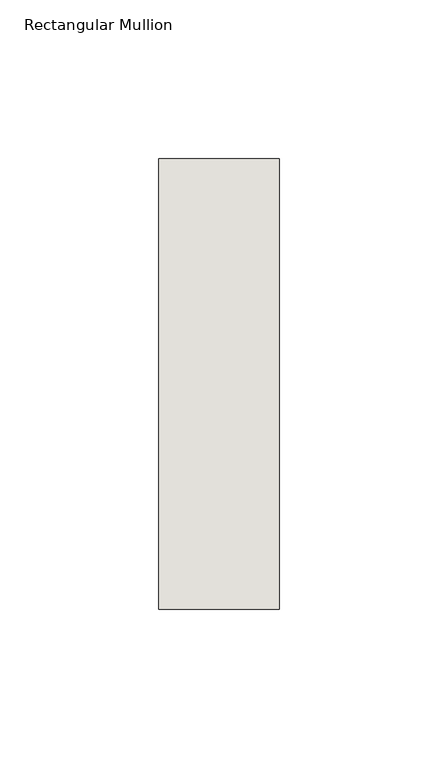
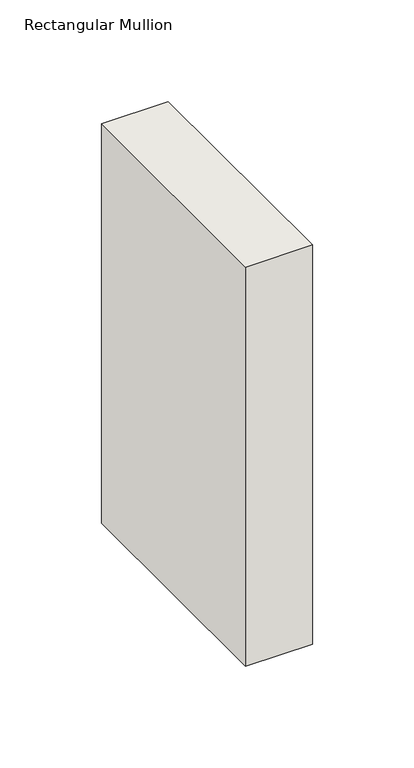
"""IFC4 building model written with IfcOpenShell, lengths in millimetres: wall geometry, Rectangular Mullion : NLRS_21_CWM_hsb-regel 38x142_gen_rsf."""

from ifc_helpers import new_model, si_unit, frame, origin, place, context, project, spatial, polyline, outline, extrude, source, transform, mapped, element, save


def rectangular_mullion_5bdfe98c(model_context):
    return source(origin(), model_context, "Body", "SweptSolid", [
        extrude(outline(polyline([(19.0, -71.0), (-19.0, -71.0), (-19.0, 71.0), (19.0, 71.0), (19.0, -71.0)])), frame((0.0, 0.0, -239.8441061), z_axis=(0.0, 0.0, 1.0), x_axis=(1.0, 0.0, 0.0)), (0.0, 0.0, 1.0), 239.8441061),
    ])


if __name__ == "__main__":
    model = new_model("IFC4")
    model_context = context("Model", 3, world=origin())
    ifc_project = project(units=[si_unit("LENGTHUNIT", "METRE", prefix="MILLI")], contexts=[model_context])
    site = spatial("IfcSite", under=ifc_project)
    building = spatial("IfcBuilding", under=site)
    placement = place(None, origin())
    rectangular_mullion_shape = rectangular_mullion_5bdfe98c(model_context)
    element("IfcWall", 1, ObjectType="Rectangular Mullion : NLRS_21_CWM_hsb-regel 38x142_gen_rsf", at=placement, inside=building, context=model_context, shape_type="MappedRepresentation", body=[
        mapped(rectangular_mullion_shape, transform((0.0, 0.0, 0.0), x_axis=(1.0, 0.0, 0.0), y_axis=(0.0, 1.0, 0.0), z_axis=(0.0, 0.0, 1.0))),
    ])
    save(model, "model.ifc")

# Revit data of these elements
# Type "Rectangular Mullion : NLRS_21_CWM_hsb-regel 38x142_gen_rsf"
#   Type IfcGUID = "07M7mRoiH1CR8m_RSKIwpF"
#   Assembly Code = "21.10"
#   IfcExportAs = "IfcWall"
#   built-in parameter 1007322 = 0.465879 (stored number, unit not read)
#   built-in parameter 1007321 = 0.062336 (stored number, unit not read)
#   built-in parameter 1007320 = 0.062336 (stored number, unit not read)
# Element 1 (IfcWall, "Rectangular Mullion : NLRS_21_CWM_hsb-regel 38x142_gen_rsf")
#   Materials on its faces: "NLRS_i2_hout naaldhout vuren_gen_rsf"
# Materials
#   "NLRS_i2_hout naaldhout vuren_gen_rsf": class "I - Hout", colour RGB 234 199 147, transparency 0, Keynote = "i2", Manufacturer = "Revit Standards Foundation", URL = "www.revitstandards.org", Description = "hout vuren", Cost = 0
